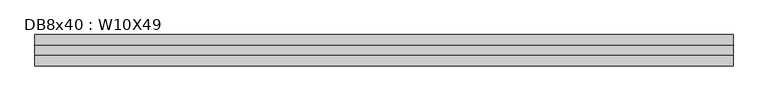
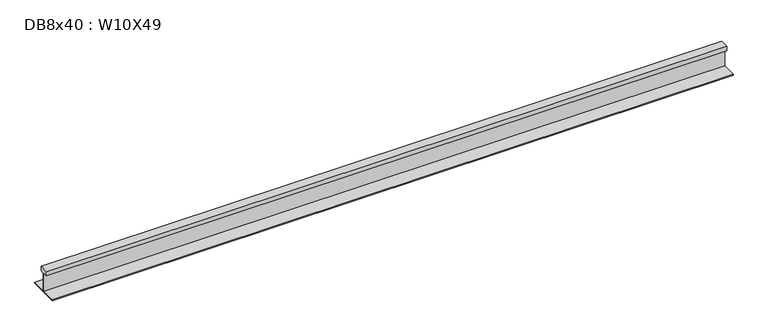
"""IFC4 building model written with IfcOpenShell, lengths in millimetres: beam geometry, DB8x40 : W10X49."""

from ifc_helpers import new_model, si_unit, frame, origin, place, context, project, spatial, polyline, outline, extrude, source, transform, mapped, element, save


def db8x40_w10x49_53ff85f1(model_context):
    return source(origin(), model_context, "Body", "SweptSolid", [
        extrude(outline(polyline([(38.1, 144.3355), (38.1, 106.2355), (2.921, 106.2355), (2.921, -49.53), (127.0, -49.53), (127.0, -59.182), (-127.0, -59.182), (-127.0, -49.53), (-2.921, -49.53), (-2.921, 106.2355), (-38.1, 106.2355), (-38.1, 144.3355), (38.1, 144.3355)])), frame((-2909.5339711, 0.0, 0.0), z_axis=(1.0, 0.0, 0.0), x_axis=(0.0, 1.0, 0.0)), (0.0, 0.0, 1.0), 5675.3519608),
    ])


if __name__ == "__main__":
    model = new_model("IFC4")
    model_context = context("Model", 3, world=origin())
    ifc_project = project(units=[si_unit("LENGTHUNIT", "METRE", prefix="MILLI")], contexts=[model_context])
    site = spatial("IfcSite", under=ifc_project)
    building = spatial("IfcBuilding", under=site)
    placement = place(None, origin())
    db8x40_w10x49_shape = db8x40_w10x49_53ff85f1(model_context)
    element("IfcBeam", 1, ObjectType="DB8x40 : W10X49", at=placement, inside=building, context=model_context, shape_type="MappedRepresentation", body=[
        mapped(db8x40_w10x49_shape, transform((0.0, 0.0, 0.0), x_axis=(1.0, 0.0, 0.0), y_axis=(0.0, 1.0, 0.0), z_axis=(0.0, 0.0, 1.0))),
    ])
    save(model, "model.ifc")

# Revit data of these elements
# Type "DB8x40 : W10X49"
#   Assembly Code = "B10"
#   W = 53
#   Length [instance default] = 5' - 0"
#   bf = 0' - 10"
#   d = 1' - 0.1"
#   k = 0' - 1 3/8"
#   k2 = 0' - 0.8"
#   tf = 0' - 0.575"
#   tw = 0' - 0.345"
#   A = 0.108333 SF
#   Structural Material [instance default] = Steel ASTM A992
# Element 1 (IfcBeam, "DB8x40 : W10X49")
#   Materials on its faces: "Steel ASTM A992"
# Materials
#   "Steel ASTM A992": class "Metal", colour RGB 199 199 199, transparency 0, Description = "Structural steel 50ksi", Cost = 0
